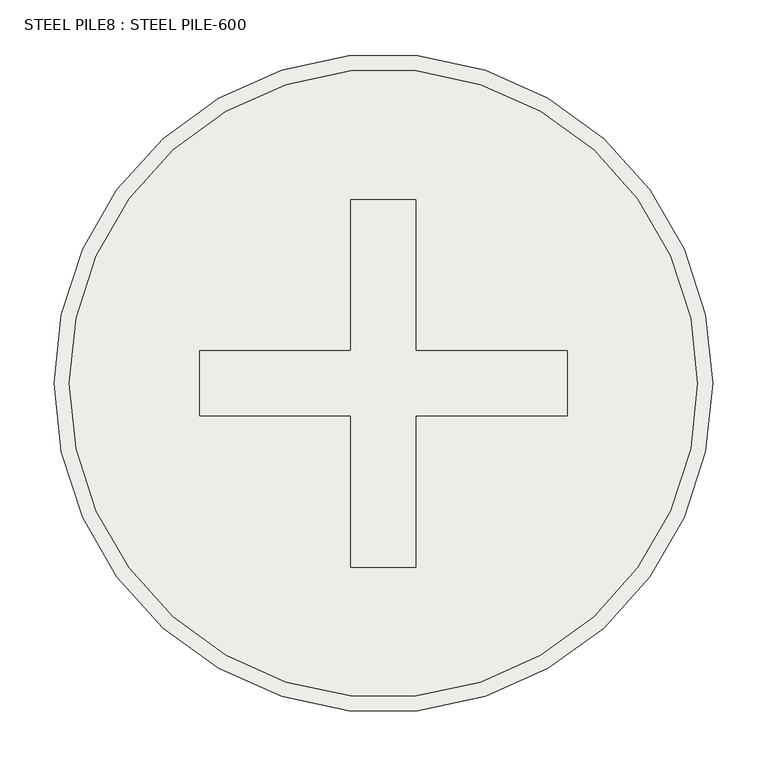
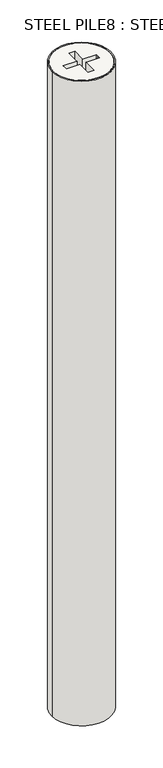
"""IFC4 building model written with IfcOpenShell, lengths in millimetres: slab geometry, STEEL PILE8 : STEEL PILE-600."""

from ifc_helpers import new_model, si_unit, point, frame, frame_2d, origin, place, context, project, spatial, circle_curve, trimmed, segment, composite_curve, outline, extrude, source, transform, mapped, element, save
from ifc_brep_helpers import plane_surface, cylinder_surface, advanced_brep


def steel_pile8_steel_pile_600_5d7a61f9(model_context):
    return source(origin(), model_context, "Body", "SolidModel", [
        advanced_brep(
        [(14709.5, 25499.5208589, 150.0), (15290.5, 25499.5208589, 150.0), (14970.0, 25469.5208589, 150.0), (14830.0, 25469.5208589, 150.0), (14830.0, 25499.5208589, 150.0), (14830.0, 25529.5208589, 150.0), (14970.0, 25529.5208589, 150.0), (14970.0, 25669.5208589, 150.0), (15030.0, 25669.5208589, 150.0), (15030.0, 25529.5208589, 150.0), (15170.0, 25529.5208589, 150.0), (15170.0, 25499.5208589, 150.0), (15170.0, 25469.5208589, 150.0), (15030.0, 25469.5208589, 150.0), (15030.0, 25329.5208589, 150.0), (14970.0, 25329.5208589, 150.0), (14709.5, 25499.5208589, -1850.0), (15290.5, 25499.5208589, -1850.0), (14830.0, 25469.5208589, -160.0), (14970.0, 25469.5208589, -160.0), (14970.0, 25329.5208589, -160.0), (15030.0, 25329.5208589, -160.0), (15030.0, 25469.5208589, -160.0), (15170.0, 25469.5208589, -160.0), (15170.0, 25499.5208589, -160.0), (15170.0, 25529.5208589, -160.0), (15030.0, 25529.5208589, -160.0), (15030.0, 25669.5208589, -160.0), (14970.0, 25669.5208589, -160.0), (14970.0, 25529.5208589, -160.0), (14830.0, 25529.5208589, -160.0), (14830.0, 25499.5208589, -160.0)],
        [
            (0, 1, circle_curve(frame((15000.0, 25499.5208589, 150.0), z_axis=(0.0, 0.0, 1.0), x_axis=(1.0, 0.0, 0.0)), 290.5)),
            (1, 0, circle_curve(frame((15000.0, 25499.5208589, 150.0), z_axis=(0.0, 0.0, 1.0), x_axis=(1.0, 0.0, 0.0)), 290.5)),
            (2, 3),
            (3, 4),
            (4, 5),
            (5, 6),
            (6, 7),
            (7, 8),
            (8, 9),
            (9, 10),
            (10, 11),
            (11, 12),
            (12, 13),
            (13, 14),
            (14, 15),
            (15, 2),
            (16, 17, circle_curve(frame((15000.0, 25499.5208589, -1850.0), z_axis=(0.0, 0.0, -1.0), x_axis=(1.0, 0.0, 0.0)), 290.5)),
            (17, 16, circle_curve(frame((15000.0, 25499.5208589, -1850.0), z_axis=(0.0, 0.0, -1.0), x_axis=(1.0, 0.0, 0.0)), 290.5)),
            (0, 16),
            (17, 1),
            (18, 19),
            (19, 20),
            (20, 21),
            (21, 22),
            (22, 23),
            (23, 24),
            (24, 25),
            (25, 26),
            (26, 27),
            (27, 28),
            (28, 29),
            (29, 30),
            (30, 31),
            (31, 18),
            (18, 3),
            (2, 19),
            (15, 20),
            (14, 21),
            (13, 22),
            (12, 23),
            (11, 24),
            (10, 25),
            (9, 26),
            (8, 27),
            (7, 28),
            (6, 29),
            (5, 30),
            (4, 31),
        ],
        [
            plane_surface(frame((15290.5, 25499.5208589, 150.0), z_axis=(0.0, 0.0, 1.0), x_axis=(0.0, 1.0, 0.0))),
            plane_surface(frame((15290.5, 25499.5208589, -1850.0), z_axis=(0.0, 0.0, -1.0), x_axis=(0.0, -1.0, 0.0))),
            cylinder_surface(frame((15000.0, 25499.5208589, -1850.0), z_axis=(0.0, 0.0, 1.0), x_axis=(1.0, 0.0, 0.0)), 290.5),
            plane_surface(frame((14830.0, 25469.5208589, -160.0), z_axis=(0.0, 0.0, 1.0), x_axis=(-1.0, 0.0, 0.0))),
            plane_surface(frame((14830.0, 25469.5208589, 160.0), z_axis=(0.0, 1.0, 0.0), x_axis=(0.0, 0.0, -1.0))),
            plane_surface(frame((14970.0, 25469.5208589, 160.0), z_axis=(1.0, 0.0, 0.0), x_axis=(0.0, 0.0, -1.0))),
            plane_surface(frame((14970.0, 25329.5208589, 160.0), z_axis=(0.0, 1.0, 0.0), x_axis=(0.0, 0.0, -1.0))),
            plane_surface(frame((15030.0, 25329.5208589, 160.0), z_axis=(-1.0, 0.0, 0.0), x_axis=(0.0, 0.0, -1.0))),
            plane_surface(frame((15030.0, 25469.5208589, 160.0), z_axis=(0.0, 1.0, 0.0), x_axis=(0.0, 0.0, -1.0))),
            plane_surface(frame((15170.0, 25469.5208589, 160.0), z_axis=(-1.0, 0.0, 0.0), x_axis=(0.0, 0.0, -1.0))),
            plane_surface(frame((15170.0, 25499.5208589, 160.0), z_axis=(-1.0, 0.0, 0.0), x_axis=(0.0, 0.0, -1.0))),
            plane_surface(frame((15170.0, 25529.5208589, 160.0), z_axis=(0.0, -1.0, 0.0), x_axis=(0.0, 0.0, -1.0))),
            plane_surface(frame((15030.0, 25529.5208589, 160.0), z_axis=(-1.0, 0.0, 0.0), x_axis=(0.0, 0.0, -1.0))),
            plane_surface(frame((15030.0, 25669.5208589, 160.0), z_axis=(0.0, -1.0, 0.0), x_axis=(0.0, 0.0, -1.0))),
            plane_surface(frame((14970.0, 25669.5208589, 160.0), z_axis=(1.0, 0.0, 0.0), x_axis=(0.0, 0.0, -1.0))),
            plane_surface(frame((14970.0, 25529.5208589, 160.0), z_axis=(0.0, -1.0, 0.0), x_axis=(0.0, 0.0, -1.0))),
            plane_surface(frame((14830.0, 25529.5208589, 160.0), z_axis=(1.0, 0.0, 0.0), x_axis=(0.0, 0.0, -1.0))),
            plane_surface(frame((14830.0, 25499.5208589, 160.0), z_axis=(1.0, 0.0, 0.0), x_axis=(0.0, 0.0, -1.0))),
        ],
        [
            (0, [[1, 2], [3, 4, 5, 6, 7, 8, 9, 10, 11, 12, 13, 14, 15, 16]]),
            (1, [[17, 18]]),
            (2, [[-1, 19, -18, 20]]),
            (2, [[-2, -20, -17, -19]]),
            (3, [[21, 22, 23, 24, 25, 26, 27, 28, 29, 30, 31, 32, 33, 34]]),
            (4, [[-21, 35, -3, 36]]),
            (5, [[-22, -36, -16, 37]]),
            (6, [[-23, -37, -15, 38]]),
            (7, [[-24, -38, -14, 39]]),
            (8, [[-25, -39, -13, 40]]),
            (9, [[-26, -40, -12, 41]]),
            (10, [[-27, -41, -11, 42]]),
            (11, [[-28, -42, -10, 43]]),
            (12, [[-29, -43, -9, 44]]),
            (13, [[-30, -44, -8, 45]]),
            (14, [[-31, -45, -7, 46]]),
            (15, [[-32, -46, -6, 47]]),
            (16, [[-33, -47, -5, 48]]),
            (17, [[-34, -48, -4, -35]]),
        ],
    ),
        extrude(outline(composite_curve([segment(trimmed(circle_curve(frame_2d((15000.0, 25499.5208589)), 304.5), [point((14695.5, 25499.5208589))], [point((15304.5, 25499.5208589))], False, "CARTESIAN"), True, "CONTINUOUS"), segment(trimmed(circle_curve(frame_2d((15000.0, 25499.5208589)), 304.5), [point((15304.5, 25499.5208589))], [point((14695.5, 25499.5208589))], False, "CARTESIAN"), True, "CONTINUOUS")], self_intersect=False), holes=[composite_curve([segment(trimmed(circle_curve(frame_2d((15000.0, 25499.5208589)), 290.5), [point((14709.5, 25499.5208589))], [point((15290.5, 25499.5208589))], True, "CARTESIAN"), True, "CONTINUOUS"), segment(trimmed(circle_curve(frame_2d((15000.0, 25499.5208589)), 290.5), [point((15290.5, 25499.5208589))], [point((14709.5, 25499.5208589))], True, "CARTESIAN"), True, "CONTINUOUS")], self_intersect=False)]), frame((0.0, 0.0, -6850.0), z_axis=(0.0, 0.0, 1.0), x_axis=(1.0, 0.0, 0.0)), (0.0, 0.0, 1.0), 7000.0),
    ])


if __name__ == "__main__":
    model = new_model("IFC4")
    model_context = context("Model", 3, world=origin())
    ifc_project = project(units=[si_unit("LENGTHUNIT", "METRE", prefix="MILLI")], contexts=[model_context])
    site = spatial("IfcSite", under=ifc_project)
    building = spatial("IfcBuilding", under=site)
    placement = place(None, origin())
    steel_pile8_steel_pile_600_shape = steel_pile8_steel_pile_600_5d7a61f9(model_context)
    element("IfcSlab", 1, ObjectType="STEEL PILE8 : STEEL PILE-600", at=placement, inside=building, context=model_context, shape_type="MappedRepresentation", body=[
        mapped(steel_pile8_steel_pile_600_shape, transform((0.0, 0.0, 0.0), x_axis=(1.0, 0.0, 0.0), y_axis=(0.0, 1.0, 0.0), z_axis=(0.0, 0.0, 1.0))),
    ])
    save(model, "model.ifc")
